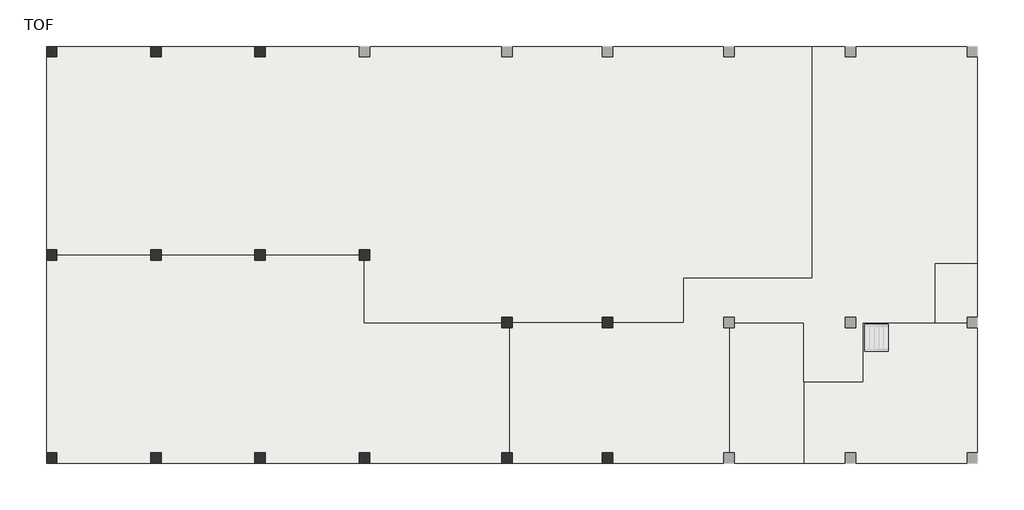
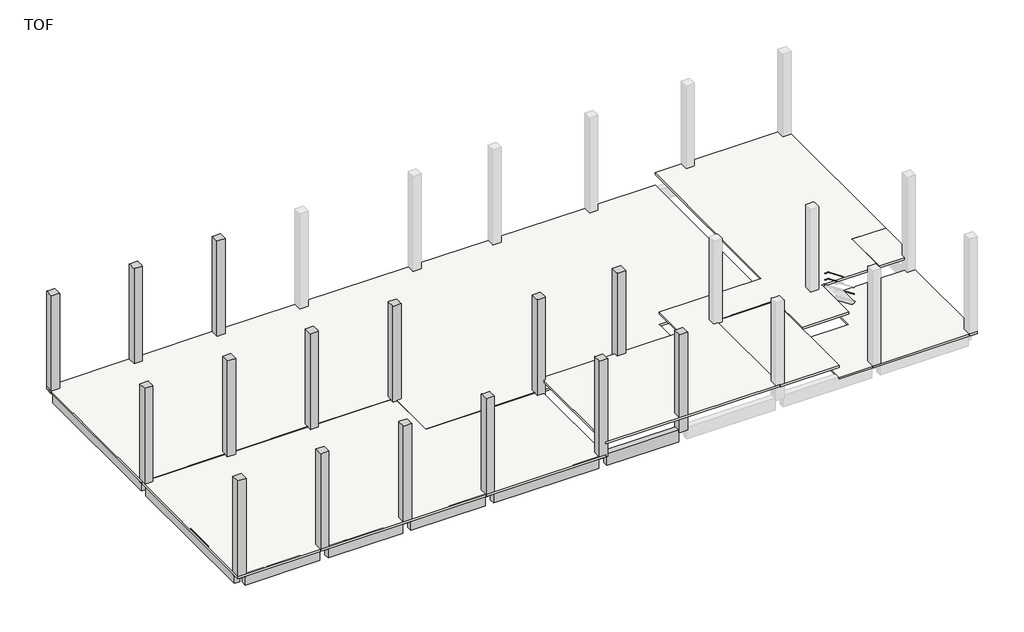
# One storey, part 1 of 2: 15 columns, 9 beams, 6 slabs.
"""IFC4 building model written with IfcOpenShell, lengths in millimetres."""

from ifc_helpers import new_model, si_unit, frame, origin, origin_with_axes, place, context, project, spatial, polyline, outline, extrude, faceted_brep, element, save

model = new_model("IFC4")

# Units and contexts
model_context = context("Model", 3, world=origin())
ifc_project = project(units=[si_unit("LENGTHUNIT", "METRE", prefix="MILLI")], contexts=[model_context])

# Site, building, storey
site = spatial("IfcSite", under=ifc_project)
building = spatial("IfcBuilding", under=site)
storey = spatial("IfcBuildingStorey", under=building, Name="TOF", Elevation=150.0)

# Beams
placement = place(None, origin())
element("IfcBeam", 1, ObjectType="RC Beam_Rectangular : H_SB_ACB_B400xH900", at=placement, inside=storey, context=model_context, shape_type="SweptSolid", body=[
    extrude(outline(polyline([(124.7, 12616.5208589), (-275.3, 12616.5208589), (-275.3, 23716.5208589), (124.7, 23716.5208589), (124.7, 12616.5208589)])), frame((0.0, 0.0, -750.0), z_axis=(0.0, 0.0, 1.0), x_axis=(1.0, 0.0, 0.0)), (0.0, 0.0, 1.0), 900.0),
])
element("IfcBeam", 2, ObjectType="RC Beam_Rectangular : H_SB_ACB_B400xH900", at=placement, inside=storey, context=model_context, shape_type="SweptSolid", body=[
    extrude(outline(polyline([(124.7, 916.5208589), (-275.3, 916.5208589), (-275.3, 12016.5208589), (124.7, 12016.5208589), (124.7, 916.5208589)])), frame((0.0, 0.0, -750.0), z_axis=(0.0, 0.0, 1.0), x_axis=(1.0, 0.0, 0.0)), (0.0, 0.0, 1.0), 900.0),
])
element("IfcBeam", 3, ObjectType="RC Beam_Rectangular : H_SB_ACB_B400xH900", at=placement, inside=storey, context=model_context, shape_type="SweptSolid", body=[
    extrude(outline(polyline([(5624.7, 24216.5208589), (5624.7, 23816.5208589), (224.7, 23816.5208589), (224.7, 24216.5208589), (5624.7, 24216.5208589)])), frame((0.0, 0.0, -750.0), z_axis=(0.0, 0.0, 1.0), x_axis=(1.0, 0.0, 0.0)), (0.0, 0.0, 1.0), 900.0),
])
element("IfcBeam", 4, ObjectType="RC Beam_Rectangular : H_SB_ACB_B400xH900", at=placement, inside=storey, context=model_context, shape_type="SweptSolid", body=[
    extrude(outline(polyline([(6224.7, 23816.5208589), (6224.7, 24216.5208589), (11624.7, 24216.5208589), (11624.7, 23816.5208589), (6224.7, 23816.5208589)])), frame((0.0, 0.0, -750.0), z_axis=(0.0, 0.0, 1.0), x_axis=(1.0, 0.0, 0.0)), (0.0, 0.0, 1.0), 900.0),
])
element("IfcBeam", 5, ObjectType="RC Beam_Rectangular : H_SB_ACB_B400xH900", at=placement, inside=storey, context=model_context, shape_type="SweptSolid", body=[
    extrude(outline(polyline([(224.7, 416.5208589), (224.7, 816.5208589), (5624.7, 816.5208589), (5624.7, 416.5208589), (224.7, 416.5208589)])), frame((0.0, 0.0, -750.0), z_axis=(0.0, 0.0, 1.0), x_axis=(1.0, 0.0, 0.0)), (0.0, 0.0, 1.0), 900.0),
])
element("IfcBeam", 6, ObjectType="RC Beam_Rectangular : H_SB_ACB_B400xH900", at=placement, inside=storey, context=model_context, shape_type="SweptSolid", body=[
    extrude(outline(polyline([(6224.7, 416.5208589), (6224.7, 816.5208589), (11624.7, 816.5208589), (11624.7, 416.5208589), (6224.7, 416.5208589)])), frame((0.0, 0.0, -750.0), z_axis=(0.0, 0.0, 1.0), x_axis=(1.0, 0.0, 0.0)), (0.0, 0.0, 1.0), 900.0),
])
element("IfcBeam", 7, ObjectType="RC Beam_Rectangular : H_SB_ACB_B400xH900", at=placement, inside=storey, context=model_context, shape_type="SweptSolid", body=[
    extrude(outline(polyline([(12224.7, 416.5208589), (12224.7, 816.5208589), (17624.7, 816.5208589), (17624.7, 416.5208589), (12224.7, 416.5208589)])), frame((0.0, 0.0, -750.0), z_axis=(0.0, 0.0, 1.0), x_axis=(1.0, 0.0, 0.0)), (0.0, 0.0, 1.0), 900.0),
])
element("IfcBeam", 8, ObjectType="RC Beam_Rectangular : H_SB_ACB_B400xH900", at=placement, inside=storey, context=model_context, shape_type="SweptSolid", body=[
    extrude(outline(polyline([(18224.7, 416.5208589), (18224.7, 816.5208589), (25824.7, 816.5208589), (25824.7, 416.5208589), (18224.7, 416.5208589)])), frame((0.0, 0.0, -750.0), z_axis=(0.0, 0.0, 1.0), x_axis=(1.0, 0.0, 0.0)), (0.0, 0.0, 1.0), 900.0),
])
element("IfcBeam", 9, ObjectType="RC Beam_Rectangular : H_SB_ACB_B400xH900", at=placement, inside=storey, context=model_context, shape_type="SweptSolid", body=[
    extrude(outline(polyline([(26424.7, 416.5208589), (26424.7, 816.5208589), (31624.7, 816.5208589), (31624.7, 416.5208589), (26424.7, 416.5208589)])), frame((0.0, 0.0, -750.0), z_axis=(0.0, 0.0, 1.0), x_axis=(1.0, 0.0, 0.0)), (0.0, 0.0, 1.0), 900.0),
])

# Columns
element("IfcColumn", 10, ObjectType="RC_Column_Rectangular : H_SC_ACC_W600xL600", at=placement, inside=storey, context=model_context, shape_type="Brep", body=[
    faceted_brep([(224.7, 12616.5208589, 0.0), (224.7, 12016.5208589, 0.0), (-375.3, 12016.5208589, 0.0), (-375.3, 12616.5208589, 0.0), (224.7, 12616.5208589, 50.0), (224.7, 12316.5208589, 50.0), (224.7, 12316.5208589, 200.0), (224.7, 12616.5208589, 200.0), (224.7, 12616.5208589, 7500.0), (224.7, 12516.5208589, 7500.0), (224.7, 12116.5208589, 7500.0), (224.7, 12016.5208589, 7500.0), (124.7, 12016.5208589, 7500.0), (-275.3, 12016.5208589, 7500.0), (-375.3, 12016.5208589, 7500.0), (-375.3, 12616.5208589, 7500.0), (-375.3, 12616.5208589, 200.0), (-375.3, 12316.5208589, 200.0), (-375.3, 12316.5208589, 50.0), (-375.3, 12616.5208589, 50.0), (-275.3, 12616.5208589, 7500.0), (124.7, 12616.5208589, 7500.0)], [[[0, 1, 2, 3]], [[1, 0, 4, 5, 6, 7, 8, 9, 10, 11]], [[2, 1, 11, 12, 13, 14]], [[3, 2, 14, 15, 16, 17, 18, 19]], [[15, 20, 21, 8, 7, 16]], [[11, 10, 9, 8, 21, 20, 15, 14, 13, 12]], [[18, 5, 4, 19]], [[6, 17, 16, 7]], [[5, 18, 17, 6]], [[0, 3, 19, 4]]]),
])
element("IfcColumn", 11, ObjectType="RC_Column_Rectangular : H_SC_ACC_W600xL600", at=placement, inside=storey, context=model_context, shape_type="Brep", body=[
    faceted_brep([(6224.7, 12616.5208589, 0.0), (6224.7, 12016.5208589, 0.0), (5624.7, 12016.5208589, 0.0), (5624.7, 12616.5208589, 0.0), (6224.7, 12616.5208589, 50.0), (6224.7, 12316.5208589, 50.0), (6224.7, 12316.5208589, 200.0), (6224.7, 12616.5208589, 200.0), (6224.7, 12616.5208589, 7500.0), (6224.7, 12516.5208589, 7500.0), (6224.7, 12116.5208589, 7500.0), (6224.7, 12016.5208589, 7500.0), (6124.7, 12016.5208589, 7500.0), (5724.7, 12016.5208589, 7500.0), (5624.7, 12016.5208589, 7500.0), (5624.7, 12116.5208589, 7500.0), (5624.7, 12516.5208589, 7500.0), (5624.7, 12616.5208589, 7500.0), (5624.7, 12616.5208589, 200.0), (5624.7, 12316.5208589, 200.0), (5624.7, 12316.5208589, 50.0), (5624.7, 12616.5208589, 50.0), (5724.7, 12616.5208589, 7500.0), (6124.7, 12616.5208589, 7500.0)], [[[0, 1, 2, 3]], [[1, 0, 4, 5, 6, 7, 8, 9, 10, 11]], [[2, 1, 11, 12, 13, 14]], [[3, 2, 14, 15, 16, 17, 18, 19, 20, 21]], [[17, 22, 23, 8, 7, 18]], [[11, 10, 9, 8, 23, 22, 17, 16, 15, 14, 13, 12]], [[20, 5, 4, 21]], [[6, 19, 18, 7]], [[5, 20, 19, 6]], [[0, 3, 21, 4]]]),
])
element("IfcColumn", 12, ObjectType="RC_Column_Rectangular : H_SC_ACC_W600xL600", at=placement, inside=storey, context=model_context, shape_type="Brep", body=[
    faceted_brep([(12224.7, 12616.5208589, 0.0), (12224.7, 12016.5208589, 0.0), (11624.7, 12016.5208589, 0.0), (11624.7, 12616.5208589, 0.0), (12224.7, 12616.5208589, 50.0), (12224.7, 12316.5208589, 50.0), (12224.7, 12316.5208589, 200.0), (12224.7, 12616.5208589, 200.0), (12224.7, 12616.5208589, 7500.0), (12224.7, 12516.5208589, 7500.0), (12224.7, 12116.5208589, 7500.0), (12224.7, 12016.5208589, 7500.0), (12124.7, 12016.5208589, 7500.0), (11724.7, 12016.5208589, 7500.0), (11624.7, 12016.5208589, 7500.0), (11624.7, 12116.5208589, 7500.0), (11624.7, 12516.5208589, 7500.0), (11624.7, 12616.5208589, 7500.0), (11624.7, 12616.5208589, 200.0), (11624.7, 12316.5208589, 200.0), (11624.7, 12316.5208589, 50.0), (11624.7, 12616.5208589, 50.0), (11724.7, 12616.5208589, 7500.0), (12124.7, 12616.5208589, 7500.0)], [[[0, 1, 2, 3]], [[1, 0, 4, 5, 6, 7, 8, 9, 10, 11]], [[2, 1, 11, 12, 13, 14]], [[3, 2, 14, 15, 16, 17, 18, 19, 20, 21]], [[17, 22, 23, 8, 7, 18]], [[11, 10, 9, 8, 23, 22, 17, 16, 15, 14, 13, 12]], [[20, 5, 4, 21]], [[6, 19, 18, 7]], [[5, 20, 19, 6]], [[0, 3, 21, 4]]]),
])
element("IfcColumn", 13, ObjectType="RC_Column_Rectangular : H_SC_ACC_W600xL600", at=placement, inside=storey, context=model_context, shape_type="Brep", body=[
    faceted_brep([(18224.7, 12616.5208589, 0.0), (18224.7, 12016.5208589, 0.0), (17624.7, 12016.5208589, 0.0), (17624.7, 12616.5208589, 0.0), (18224.7, 12616.5208589, 7500.0), (18224.7, 12516.5208589, 7500.0), (18224.7, 12116.5208589, 7500.0), (18224.7, 12016.5208589, 7500.0), (18224.7, 12016.5208589, 200.0), (18224.7, 12616.5208589, 200.0), (18224.7, 12016.5208589, 50.0), (17924.7, 12016.5208589, 50.0), (17924.7, 12016.5208589, 200.0), (18124.7, 12016.5208589, 7500.0), (17724.7, 12016.5208589, 7500.0), (17624.7, 12016.5208589, 7500.0), (17624.7, 12116.5208589, 7500.0), (17624.7, 12516.5208589, 7500.0), (17624.7, 12616.5208589, 7500.0), (17624.7, 12616.5208589, 200.0), (17624.7, 12316.5208589, 200.0), (17624.7, 12316.5208589, 50.0), (17624.7, 12616.5208589, 50.0), (17724.7, 12616.5208589, 7500.0), (18124.7, 12616.5208589, 7500.0), (17924.7, 12316.5208589, 50.0), (18224.7, 12616.5208589, 50.0), (17924.7, 12316.5208589, 200.0)], [[[0, 1, 2, 3]], [[4, 5, 6, 7, 8, 9]], [[2, 1, 10, 11, 12, 8, 7, 13, 14, 15]], [[3, 2, 15, 16, 17, 18, 19, 20, 21, 22]], [[18, 23, 24, 4, 9, 19]], [[7, 6, 5, 4, 24, 23, 18, 17, 16, 15, 14, 13]], [[21, 25, 11, 10, 26, 22]], [[12, 27, 20, 19, 9, 8]], [[25, 27, 12, 11]], [[27, 25, 21, 20]], [[1, 0, 26, 10]], [[0, 3, 22, 26]]]),
])
element("IfcColumn", 14, ObjectType="RC_Column_Rectangular : H_SC_ACC_W600xL600", at=placement, inside=storey, context=model_context, shape_type="Brep", body=[
    faceted_brep([(224.7, 24316.5208589, 0.0), (224.7, 23716.5208589, 0.0), (-375.3, 23716.5208589, 0.0), (-375.3, 24316.5208589, 0.0), (224.7, 23716.5208589, 50.0), (224.7, 24316.5208589, 50.0), (-375.3, 24316.5208589, 50.0), (-375.3, 23716.5208589, 50.0)], [[[0, 1, 2, 3]], [[4, 5, 6, 7]], [[1, 0, 5, 4]], [[2, 1, 4, 7]], [[3, 2, 7, 6]], [[0, 3, 6, 5]]]),
    faceted_brep([(224.7, 24316.5208589, 7500.0), (224.7, 24216.5208589, 7500.0), (224.7, 23816.5208589, 7500.0), (224.7, 23716.5208589, 7500.0), (224.7, 23716.5208589, 200.0), (224.7, 24316.5208589, 200.0), (124.7, 23716.5208589, 7500.0), (-275.3, 23716.5208589, 7500.0), (-375.3, 23716.5208589, 7500.0), (-375.3, 23716.5208589, 200.0), (-375.3, 24316.5208589, 7500.0), (-375.3, 24316.5208589, 200.0), (-275.3, 24316.5208589, 7500.0), (124.7, 24316.5208589, 7500.0)], [[[0, 1, 2, 3, 4, 5]], [[3, 6, 7, 8, 9, 4]], [[8, 10, 11, 9]], [[10, 12, 13, 0, 5, 11]], [[3, 2, 1, 0, 13, 12, 10, 8, 7, 6]], [[5, 4, 9, 11]]]),
])
element("IfcColumn", 15, ObjectType="RC_Column_Rectangular : H_SC_ACC_W600xL600", at=placement, inside=storey, context=model_context, shape_type="Brep", body=[
    faceted_brep([(6224.7, 24316.5208589, 0.0), (6224.7, 23716.5208589, 0.0), (5624.7, 23716.5208589, 0.0), (5624.7, 24316.5208589, 0.0), (6224.7, 23716.5208589, 50.0), (6224.7, 24316.5208589, 50.0), (5624.7, 24316.5208589, 50.0), (5624.7, 23716.5208589, 50.0)], [[[0, 1, 2, 3]], [[4, 5, 6, 7]], [[1, 0, 5, 4]], [[2, 1, 4, 7]], [[3, 2, 7, 6]], [[0, 3, 6, 5]]]),
    faceted_brep([(6224.7, 24316.5208589, 7500.0), (6224.7, 24216.5208589, 7500.0), (6224.7, 23816.5208589, 7500.0), (6224.7, 23716.5208589, 7500.0), (6224.7, 23716.5208589, 200.0), (6224.7, 24316.5208589, 200.0), (6124.7, 23716.5208589, 7500.0), (5724.7, 23716.5208589, 7500.0), (5624.7, 23716.5208589, 7500.0), (5624.7, 23716.5208589, 200.0), (5624.7, 23816.5208589, 7500.0), (5624.7, 24216.5208589, 7500.0), (5624.7, 24316.5208589, 7500.0), (5624.7, 24316.5208589, 200.0), (5724.7, 24316.5208589, 7500.0), (6124.7, 24316.5208589, 7500.0)], [[[0, 1, 2, 3, 4, 5]], [[3, 6, 7, 8, 9, 4]], [[8, 10, 11, 12, 13, 9]], [[12, 14, 15, 0, 5, 13]], [[3, 2, 1, 0, 15, 14, 12, 11, 10, 8, 7, 6]], [[5, 4, 9, 13]]]),
])
element("IfcColumn", 16, ObjectType="RC_Column_Rectangular : H_SC_ACC_W600xL600", at=placement, inside=storey, context=model_context, shape_type="Brep", body=[
    faceted_brep([(12224.7, 24316.5208589, 0.0), (12224.7, 23716.5208589, 0.0), (11624.7, 23716.5208589, 0.0), (11624.7, 24316.5208589, 0.0), (12224.7, 23716.5208589, 50.0), (12224.7, 24316.5208589, 50.0), (11624.7, 24316.5208589, 50.0), (11624.7, 23716.5208589, 50.0)], [[[0, 1, 2, 3]], [[4, 5, 6, 7]], [[1, 0, 5, 4]], [[2, 1, 4, 7]], [[3, 2, 7, 6]], [[0, 3, 6, 5]]]),
    faceted_brep([(12224.7, 24316.5208589, 7500.0), (12224.7, 24216.5208589, 7500.0), (12224.7, 23816.5208589, 7500.0), (12224.7, 23716.5208589, 7500.0), (12224.7, 23716.5208589, 200.0), (12224.7, 24316.5208589, 200.0), (12124.7, 23716.5208589, 7500.0), (11724.7, 23716.5208589, 7500.0), (11624.7, 23716.5208589, 7500.0), (11624.7, 23716.5208589, 200.0), (11624.7, 23816.5208589, 7500.0), (11624.7, 24216.5208589, 7500.0), (11624.7, 24316.5208589, 7500.0), (11624.7, 24316.5208589, 200.0), (11724.7, 24316.5208589, 7500.0), (12124.7, 24316.5208589, 7500.0)], [[[0, 1, 2, 3, 4, 5]], [[3, 6, 7, 8, 9, 4]], [[8, 10, 11, 12, 13, 9]], [[12, 14, 15, 0, 5, 13]], [[3, 2, 1, 0, 15, 14, 12, 11, 10, 8, 7, 6]], [[5, 4, 9, 13]]]),
])
element("IfcColumn", 17, ObjectType="RC_Column_Rectangular : H_SC_ACC_W600xL600", at=placement, inside=storey, context=model_context, shape_type="Brep", body=[
    faceted_brep([(26424.7, 8716.5208589, 0.0), (26424.7, 8116.5208589, 0.0), (25824.7, 8116.5208589, 0.0), (25824.7, 8716.5208589, 0.0), (26424.7, 8716.5208589, 50.0), (26424.7, 8416.5208589, 50.0), (26424.7, 8416.5208589, 200.0), (26424.7, 8716.5208589, 200.0), (26424.7, 8716.5208589, 7500.0), (26424.7, 8616.5208589, 7500.0), (26424.7, 8216.5208589, 7500.0), (26424.7, 8116.5208589, 7500.0), (26324.7, 8116.5208589, 7500.0), (25924.7, 8116.5208589, 7500.0), (25824.7, 8116.5208589, 7500.0), (25824.7, 8216.5208589, 7500.0), (25824.7, 8616.5208589, 7500.0), (25824.7, 8716.5208589, 7500.0), (25824.7, 8716.5208589, 200.0), (25824.7, 8416.5208589, 200.0), (25824.7, 8416.5208589, 50.0), (25824.7, 8716.5208589, 50.0), (25924.7, 8716.5208589, 7500.0), (26324.7, 8716.5208589, 7500.0)], [[[0, 1, 2, 3]], [[1, 0, 4, 5, 6, 7, 8, 9, 10, 11]], [[2, 1, 11, 12, 13, 14]], [[3, 2, 14, 15, 16, 17, 18, 19, 20, 21]], [[17, 22, 23, 8, 7, 18]], [[11, 10, 9, 8, 23, 22, 17, 16, 15, 14, 13, 12]], [[20, 5, 4, 21]], [[6, 19, 18, 7]], [[5, 20, 19, 6]], [[0, 3, 21, 4]]]),
])
element("IfcColumn", 18, ObjectType="RC_Column_Rectangular : H_SC_ACC_W600xL600", at=placement, inside=storey, context=model_context, shape_type="Brep", body=[
    faceted_brep([(32224.7, 8716.5208589, 0.0), (32224.7, 8116.5208589, 0.0), (31624.7, 8116.5208589, 0.0), (31624.7, 8716.5208589, 0.0), (32224.7, 8716.5208589, 50.0), (32224.7, 8416.5208589, 50.0), (32224.7, 8416.5208589, 200.0), (32224.7, 8716.5208589, 200.0), (32224.7, 8716.5208589, 7500.0), (32224.7, 8616.5208589, 7500.0), (32224.7, 8216.5208589, 7500.0), (32224.7, 8116.5208589, 7500.0), (32124.7, 8116.5208589, 7500.0), (31724.7, 8116.5208589, 7500.0), (31624.7, 8116.5208589, 7500.0), (31624.7, 8216.5208589, 7500.0), (31624.7, 8616.5208589, 7500.0), (31624.7, 8716.5208589, 7500.0), (31624.7, 8716.5208589, 200.0), (31624.7, 8416.5208589, 200.0), (31624.7, 8416.5208589, 50.0), (31624.7, 8716.5208589, 50.0), (31724.7, 8716.5208589, 7500.0), (32124.7, 8716.5208589, 7500.0)], [[[0, 1, 2, 3]], [[1, 0, 4, 5, 6, 7, 8, 9, 10, 11]], [[2, 1, 11, 12, 13, 14]], [[3, 2, 14, 15, 16, 17, 18, 19, 20, 21]], [[17, 22, 23, 8, 7, 18]], [[11, 10, 9, 8, 23, 22, 17, 16, 15, 14, 13, 12]], [[20, 5, 4, 21]], [[6, 19, 18, 7]], [[5, 20, 19, 6]], [[0, 3, 21, 4]]]),
])
element("IfcColumn", 19, ObjectType="RC_Column_Rectangular : H_SC_ACC_W600xL600", at=placement, inside=storey, context=model_context, shape_type="Brep", body=[
    faceted_brep([(224.7, 916.5208589, 0.0), (224.7, 316.5208589, 0.0), (-375.3, 316.5208589, 0.0), (-375.3, 916.5208589, 0.0), (224.7, 916.5208589, 7500.0), (224.7, 816.5208589, 7500.0), (224.7, 416.5208589, 7500.0), (224.7, 316.5208589, 7500.0), (-375.3, 316.5208589, 7500.0), (-375.3, 916.5208589, 7500.0), (-275.3, 916.5208589, 7500.0), (124.7, 916.5208589, 7500.0)], [[[0, 1, 2, 3]], [[4, 5, 6, 7, 1, 0]], [[7, 8, 2, 1]], [[8, 9, 3, 2]], [[9, 10, 11, 4, 0, 3]], [[4, 11, 10, 9, 8, 7, 6, 5]]]),
])
element("IfcColumn", 20, ObjectType="RC_Column_Rectangular : H_SC_ACC_W600xL600", at=placement, inside=storey, context=model_context, shape_type="Brep", body=[
    faceted_brep([(6224.7, 916.5208589, 0.0), (6224.7, 316.5208589, 0.0), (5624.7, 316.5208589, 0.0), (5624.7, 916.5208589, 0.0), (6224.7, 916.5208589, 7500.0), (6224.7, 816.5208589, 7500.0), (6224.7, 416.5208589, 7500.0), (6224.7, 316.5208589, 7500.0), (5624.7, 316.5208589, 7500.0), (5624.7, 416.5208589, 7500.0), (5624.7, 816.5208589, 7500.0), (5624.7, 916.5208589, 7500.0), (5724.7, 916.5208589, 7500.0), (6124.7, 916.5208589, 7500.0)], [[[0, 1, 2, 3]], [[4, 5, 6, 7, 1, 0]], [[7, 8, 2, 1]], [[8, 9, 10, 11, 3, 2]], [[11, 12, 13, 4, 0, 3]], [[4, 13, 12, 11, 10, 9, 8, 7, 6, 5]]]),
])
element("IfcColumn", 21, ObjectType="RC_Column_Rectangular : H_SC_ACC_W600xL600", at=placement, inside=storey, context=model_context, shape_type="Brep", body=[
    faceted_brep([(12224.7, 916.5208589, 0.0), (12224.7, 316.5208589, 0.0), (11624.7, 316.5208589, 0.0), (11624.7, 916.5208589, 0.0), (12224.7, 916.5208589, 7500.0), (12224.7, 816.5208589, 7500.0), (12224.7, 416.5208589, 7500.0), (12224.7, 316.5208589, 7500.0), (11624.7, 316.5208589, 7500.0), (11624.7, 416.5208589, 7500.0), (11624.7, 816.5208589, 7500.0), (11624.7, 916.5208589, 7500.0), (11724.7, 916.5208589, 7500.0), (12124.7, 916.5208589, 7500.0)], [[[0, 1, 2, 3]], [[4, 5, 6, 7, 1, 0]], [[7, 8, 2, 1]], [[8, 9, 10, 11, 3, 2]], [[11, 12, 13, 4, 0, 3]], [[4, 13, 12, 11, 10, 9, 8, 7, 6, 5]]]),
])
element("IfcColumn", 22, ObjectType="RC_Column_Rectangular : H_SC_ACC_W600xL600", at=placement, inside=storey, context=model_context, shape_type="Brep", body=[
    faceted_brep([(18224.7, 916.5208589, 0.0), (18224.7, 316.5208589, 0.0), (17624.7, 316.5208589, 0.0), (17624.7, 916.5208589, 0.0), (18224.7, 916.5208589, 7500.0), (18224.7, 816.5208589, 7500.0), (18224.7, 416.5208589, 7500.0), (18224.7, 316.5208589, 7500.0), (17624.7, 316.5208589, 7500.0), (17624.7, 416.5208589, 7500.0), (17624.7, 816.5208589, 7500.0), (17624.7, 916.5208589, 7500.0), (17724.7, 916.5208589, 7500.0), (18124.7, 916.5208589, 7500.0)], [[[0, 1, 2, 3]], [[4, 5, 6, 7, 1, 0]], [[7, 8, 2, 1]], [[8, 9, 10, 11, 3, 2]], [[11, 12, 13, 4, 0, 3]], [[4, 13, 12, 11, 10, 9, 8, 7, 6, 5]]]),
])
element("IfcColumn", 23, ObjectType="RC_Column_Rectangular : H_SC_ACC_W600xL600", at=placement, inside=storey, context=model_context, shape_type="Brep", body=[
    faceted_brep([(26424.7, 916.5208589, 0.0), (26424.7, 316.5208589, 0.0), (25824.7, 316.5208589, 0.0), (25824.7, 916.5208589, 0.0), (26424.7, 916.5208589, 7500.0), (26424.7, 816.5208589, 7500.0), (26424.7, 416.5208589, 7500.0), (26424.7, 316.5208589, 7500.0), (25824.7, 316.5208589, 7500.0), (25824.7, 416.5208589, 7500.0), (25824.7, 816.5208589, 7500.0), (25824.7, 916.5208589, 7500.0), (25924.7, 916.5208589, 7500.0), (26324.7, 916.5208589, 7500.0)], [[[0, 1, 2, 3]], [[4, 5, 6, 7, 1, 0]], [[7, 8, 2, 1]], [[8, 9, 10, 11, 3, 2]], [[11, 12, 13, 4, 0, 3]], [[4, 13, 12, 11, 10, 9, 8, 7, 6, 5]]]),
])
element("IfcColumn", 24, ObjectType="RC_Column_Rectangular : H_SC_ACC_W600xL600", at=placement, inside=storey, context=model_context, shape_type="Brep", body=[
    faceted_brep([(32224.7, 916.5208589, 0.0), (32224.7, 316.5208589, 0.0), (31624.7, 316.5208589, 0.0), (31624.7, 916.5208589, 0.0), (32224.7, 916.5208589, 7500.0), (32224.7, 816.5208589, 7500.0), (32224.7, 416.5208589, 7500.0), (32224.7, 316.5208589, 7500.0), (31624.7, 316.5208589, 7500.0), (31624.7, 416.5208589, 7500.0), (31624.7, 816.5208589, 7500.0), (31624.7, 916.5208589, 7500.0), (31724.7, 916.5208589, 7500.0), (32124.7, 916.5208589, 7500.0)], [[[0, 1, 2, 3]], [[4, 5, 6, 7, 1, 0]], [[7, 8, 2, 1]], [[8, 9, 10, 11, 3, 2]], [[11, 12, 13, 4, 0, 3]], [[4, 13, 12, 11, 10, 9, 8, 7, 6, 5]]]),
])

# Slabs
element("IfcSlab", 25, ObjectType="H_FL_AMF_RC Slab_T150", at=placement, inside=storey, context=model_context, shape_type="Brep", body=[
    faceted_brep([(-375.3, 24316.5208589, 50.0), (224.7, 24316.5208589, 50.0), (5624.7, 24316.5208589, 50.0), (6224.7, 24316.5208589, 50.0), (11624.7, 24316.5208589, 50.0), (12224.7, 24316.5208589, 50.0), (17624.7, 24316.5208589, 50.0), (18224.7, 24316.5208589, 50.0), (25824.7, 24316.5208589, 50.0), (26424.7, 24316.5208589, 50.0), (31624.7, 24316.5208589, 50.0), (32224.7, 24316.5208589, 50.0), (38624.7, 24316.5208589, 50.0), (39224.7, 24316.5208589, 50.0), (43724.7, 24316.5208589, 50.0), (43724.7, 10966.5208589, 50.0), (36324.7, 10966.5208589, 50.0), (36324.7, 8416.5208589, 50.0), (32224.7, 8416.5208589, 50.0), (31624.7, 8416.5208589, 50.0), (26424.7, 8416.5208589, 50.0), (25824.7, 8416.5208589, 50.0), (17924.7, 8416.5208589, 50.0), (17924.7, 12016.5208589, 50.0), (17924.7, 12316.5208589, 50.0), (17624.7, 12316.5208589, 50.0), (12224.7, 12316.5208589, 50.0), (11624.7, 12316.5208589, 50.0), (6224.7, 12316.5208589, 50.0), (5624.7, 12316.5208589, 50.0), (224.7, 12316.5208589, 50.0), (-375.3, 12316.5208589, 50.0), (-375.3, 12616.5208589, 50.0), (-375.3, 23716.5208589, 50.0), (-375.3, 24316.5208589, 200.0), (-375.3, 23716.5208589, 200.0), (-375.3, 12616.5208589, 200.0), (-375.3, 12316.5208589, 200.0), (224.7, 12316.5208589, 200.0), (5624.7, 12316.5208589, 200.0), (6224.7, 12316.5208589, 200.0), (11624.7, 12316.5208589, 200.0), (12224.7, 12316.5208589, 200.0), (17624.7, 12316.5208589, 200.0), (17924.7, 12316.5208589, 200.0), (17924.7, 12016.5208589, 200.0), (17924.7, 8416.5208589, 200.0), (25824.7, 8416.5208589, 200.0), (26424.7, 8416.5208589, 200.0), (31624.7, 8416.5208589, 200.0), (32224.7, 8416.5208589, 200.0), (36324.7, 8416.5208589, 200.0), (36324.7, 10966.5208589, 200.0), (43724.7, 10966.5208589, 200.0), (43724.7, 24316.5208589, 200.0), (39224.7, 24316.5208589, 200.0), (38624.7, 24316.5208589, 200.0), (32224.7, 24316.5208589, 200.0), (31624.7, 24316.5208589, 200.0), (26424.7, 24316.5208589, 200.0), (25824.7, 24316.5208589, 200.0), (18224.7, 24316.5208589, 200.0), (17624.7, 24316.5208589, 200.0), (12224.7, 24316.5208589, 200.0), (11624.7, 24316.5208589, 200.0), (6224.7, 24316.5208589, 200.0), (5624.7, 24316.5208589, 200.0), (224.7, 24316.5208589, 200.0)], [[[0, 1, 2, 3, 4, 5, 6, 7, 8, 9, 10, 11, 12, 13, 14, 15, 16, 17, 18, 19, 20, 21, 22, 23, 24, 25, 26, 27, 28, 29, 30, 31, 32, 33]], [[34, 35, 36, 37, 38, 39, 40, 41, 42, 43, 44, 45, 46, 47, 48, 49, 50, 51, 52, 53, 54, 55, 56, 57, 58, 59, 60, 61, 62, 63, 64, 65, 66, 67]], [[0, 33, 32, 31, 37, 36, 35, 34]], [[14, 13, 12, 11, 10, 9, 8, 7, 6, 5, 4, 3, 2, 1, 0, 34, 67, 66, 65, 64, 63, 62, 61, 60, 59, 58, 57, 56, 55, 54]], [[15, 14, 54, 53]], [[16, 15, 53, 52]], [[17, 16, 52, 51]], [[22, 21, 20, 19, 18, 17, 51, 50, 49, 48, 47, 46]], [[24, 23, 22, 46, 45, 44]], [[31, 30, 29, 28, 27, 26, 25, 24, 44, 43, 42, 41, 40, 39, 38, 37]]]),
])
element("IfcSlab", 26, ObjectType="H_FL_AMF_RC Slab_T150", at=placement, inside=storey, context=model_context, shape_type="SweptSolid", body=[
    extrude(outline(polyline([(53224.7, 11850.5208589), (50777.7, 11850.5208589), (50777.7, 8416.5208589), (46624.7, 8416.5208589), (46624.7, 5013.5208589), (43224.7, 5013.5208589), (43224.7, 8416.5208589), (38924.7, 8416.5208589), (38924.7, 316.5208589), (26307.7, 316.5208589), (26307.7, 8416.5208589), (36324.7, 8416.5208589), (36324.7, 10966.5208589), (43724.7, 10966.5208589), (43724.7, 24316.5208589), (53224.7, 24316.5208589), (53224.7, 11850.5208589)])), frame((0.0, 0.0, 1000.0), z_axis=(0.0, 0.0, 1.0), x_axis=(1.0, 0.0, 0.0)), (0.0, 0.0, 1.0), 150.0),
])
element("IfcSlab", 27, ObjectType="H_FL_AMF_RC Slab_T150", at=placement, inside=storey, context=model_context, shape_type="SweptSolid", body=[
    extrude(outline(polyline([(17924.7, 12316.5208589), (17924.7, 8416.5208589), (26307.7, 8416.5208589), (26307.7, 316.5208589), (-375.3, 316.5208589), (-375.3, 12316.5208589), (17924.7, 12316.5208589)])), origin_with_axes(), (0.0, 0.0, 1.0), 150.0),
])
element("IfcSlab", 28, ObjectType="H_FL_AMF_RC Slab_T150", at=placement, inside=storey, context=model_context, shape_type="SweptSolid", body=[
    extrude(outline(polyline([(53224.7, 11850.5208589), (53224.7, 8416.5208589), (50777.7, 8416.5208589), (50777.7, 11850.5208589), (53224.7, 11850.5208589)])), frame((0.0, 0.0, 1000.0), z_axis=(0.0, 0.0, 1.0), x_axis=(1.0, 0.0, 0.0)), (0.0, 0.0, 1.0), 150.0),
])
element("IfcSlab", 29, ObjectType="H_FL_AMF_RC Slab_T150", at=placement, inside=storey, context=model_context, shape_type="SweptSolid", body=[
    extrude(outline(polyline([(46624.7, 8416.5208589), (53224.7, 8416.5208589), (53224.7, 316.5208589), (43224.7, 316.5208589), (43224.7, 5018.5208589), (46624.7, 5018.5208589), (46624.7, 8416.5208589)])), frame((0.0, 0.0, 50.0), z_axis=(0.0, 0.0, 1.0), x_axis=(1.0, 0.0, 0.0)), (0.0, 0.0, 1.0), 150.0),
])
element("IfcSlab", 30, ObjectType="H_FL_AMF_RC Slab_T150", at=placement, inside=storey, context=model_context, shape_type="SweptSolid", body=[
    extrude(outline(polyline([(38924.7, 316.5208589), (38924.7, 8416.5208589), (43224.7, 8416.5208589), (43224.7, 316.5208589), (38924.7, 316.5208589)])), frame((0.0, 0.0, 950.0), z_axis=(0.0, 0.0, 1.0), x_axis=(1.0, 0.0, 0.0)), (0.0, 0.0, 1.0), 150.0),
])

save(model, "model.ifc")

# Revit data of these elements
# Project information
#   Building Name = "SULFUR LOADING CONTROL BD"
#   Project Status = "Project Status"
#   Client Name = "현대엔지니어링"
#   Project Address = "서울시 종로구 율곡로 75(계동)"
#   Project Number = "-"
# Grids (mm)
#   "Y1": line (-3935.398, 24016.521) -> (58968.688, 24016.521)
#   "X1": line (-75.3, 29394.337) -> (-75.3, -4379.638)
#   "X2": line (5924.7, 29394.337) -> (5924.7, -4379.638)
#   "Y3": line (-3935.398, 8416.521) -> (58968.688, 8416.521)
#   "Y4": line (-3935.398, 616.521) -> (58968.688, 616.521)
#   "X3": line (11924.7, 29394.337) -> (11924.7, -4379.638)
#   "X4": line (17924.7, 29394.337) -> (17924.7, -4379.638)
#   "X5": line (26124.7, 29394.337) -> (26124.7, -4379.638)
#   "X6": line (31924.7, 29394.337) -> (31924.7, -4379.638)
#   "X7": line (38924.7, 29394.337) -> (38924.7, -4379.638)
#   "X8": line (45924.7, 29394.337) -> (45924.7, -4379.638)
#   "X9": line (52924.7, 29394.337) -> (52924.7, -4379.638)
#   "X15": line (43724.7, 27041.858) -> (43724.7, 9156.488)
#   "X16": line (36324.7, 27041.858) -> (36324.7, 9156.488)
#   "X17": line (34685.051, 10966.521) -> (55094.626, 10966.521)
#   "X18": line (34685.051, 18666.521) -> (55094.626, 18666.521)
#   "Y2": line (-3935.398, 12316.521) -> (58968.688, 12316.521)
# Type "RC Beam_Rectangular : H_SB_ACB_B400xH900"
#   중앙부 하부근 = ""
#   중앙부 상부근 = ""
#   중앙부 보조근 = ""
#   중앙부 늑근 = ""
#   외단부 하부근 = ""
#   외단부 상부근 = ""
#   외단부 보조근 = ""
#   외단부 늑근 = ""
#   부호 = "TG3"
#   내단부 하부근 = ""
#   내단부 상부근 = ""
#   내단부 보조근 = ""
#   내단부 늑근 = ""
#   ALL 하부근 = "3-D20"
#   ALL 상부근 = "3-D20"
#   ALL 보조근 = ""
#   ALL 늑근 = "2-D10 @120"
#   Width = 400.000 mm
#   Height = 900.000 mm
#   Length [instance default] = 1524.000 mm
#   b = 400.000 mm
#   h = 900.000 mm
#   hec_material3 [instance default] = none
#   hec_material2 [instance default] = none
#   hec_material1 [instance default] = none
#   Structural Material [instance default] = none
#   Assembly Code = ""
# Type "RC_Column_Rectangular : H_SC_ACC_W600xL600"
#   Width = 600.000 mm
#   Length = 600.000 mm
#   hec_material3 [instance default] = none
#   hec_material2 [instance default] = none
#   hec_material1 [instance default] = none
#   Structural Material [instance default] = none
#   Description = (empty or 0)
# Type "H_FL_AMF_RC Slab_T150"
#   Keynote = ""
#   Type Comments = ""
#   Description = ""
#   Function = 1
#   Layers, outside or top first: 150.000 mm no material (function 1)
# Elements 1, 2, 3, 4, 5, 6, 7, 8, 9 (IfcBeam, "RC Beam_Rectangular : H_SB_ACB_B400xH900")
#   hec_material3 = none
#   hec_material2 = none
#   hec_material1 = none
#   Structural Material = none
#   Phase Created = New Construction
# Elements 10, 11, 12, 13, 14, 15, 16, 17, 18, 19, 20, 21, 22, 23, 24 (IfcColumn, "RC_Column_Rectangular : H_SC_ACC_W600xL600")
#   Comments = ""
#   hec_material3 = none
#   hec_material2 = none
#   hec_material1 = none
#   Structural Material = none
#   Phase Created = New Construction
# Element 25 (IfcSlab, "H_FL_AMF_RC Slab_T150")
#   Height Offset From Level = 50.000 mm
#   Phase Created = New Construction
#   Materials on its faces: "Default Floor"
# Elements 26, 28 (IfcSlab, "H_FL_AMF_RC Slab_T150")
#   Height Offset From Level = 1000.000 mm
#   Phase Created = New Construction
#   Materials on its faces: "Default Floor"
# Element 27 (IfcSlab, "H_FL_AMF_RC Slab_T150")
#   built-in parameter 1001955 = 1.5708 (stored number, unit not read)
#   Height Offset From Level = 0.000 mm
#   Phase Created = New Construction
#   Materials on its faces: "Default Floor"
# Element 29 (IfcSlab, "H_FL_AMF_RC Slab_T150")
#   built-in parameter 1001955 = 3.14159 (stored number, unit not read)
#   Height Offset From Level = 50.000 mm
#   Phase Created = New Construction
#   Materials on its faces: "Default Floor"
# Element 30 (IfcSlab, "H_FL_AMF_RC Slab_T150")
#   built-in parameter 1001955 = -1.5708 (stored number, unit not read)
#   Height Offset From Level = 950.000 mm
#   Phase Created = New Construction
#   Materials on its faces: "Default Floor"
# Materials
#   "Default Floor": class "Miscellaneous", colour RGB 80 80 80, transparency 0
